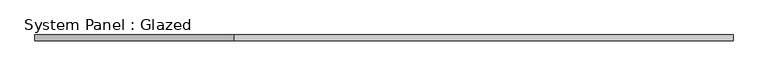
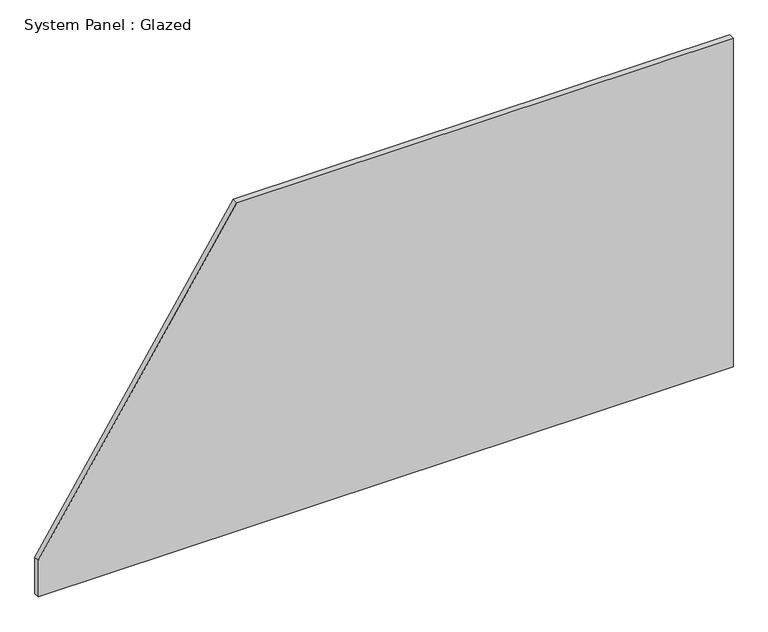
"""IFC4 building model written with IfcOpenShell, lengths in millimetres: plate geometry, System Panel : Glazed."""

from ifc_helpers import new_model, si_unit, frame, origin, place, context, project, spatial, polyline, outline, extrude, source, transform, mapped, element, save


def system_panel_glazed_b6f49b0a(model_context):
    return source(origin(), model_context, "Body", "SweptSolid", [
        extrude(outline(polyline([(0.0, -1500.0), (0.0, 1500.0), (1500.0, 1500.0), (1500.0, -642.8120991), (166.61217, -1500.0), (0.0, -1500.0)])), frame((0.0, 24.5, 0.0), z_axis=(0.0, 1.0, 0.0), x_axis=(0.0, 0.0, 1.0)), (0.0, 0.0, 1.0), 25.0),
    ])


if __name__ == "__main__":
    model = new_model("IFC4")
    model_context = context("Model", 3, world=origin())
    ifc_project = project(units=[si_unit("LENGTHUNIT", "METRE", prefix="MILLI")], contexts=[model_context])
    site = spatial("IfcSite", under=ifc_project)
    building = spatial("IfcBuilding", under=site)
    placement = place(None, origin())
    system_panel_glazed_shape = system_panel_glazed_b6f49b0a(model_context)
    element("IfcPlate", 1, ObjectType="System Panel : Glazed", at=placement, inside=building, context=model_context, shape_type="MappedRepresentation", body=[
        mapped(system_panel_glazed_shape, transform((0.0, 0.0, 0.0), x_axis=(1.0, 0.0, 0.0), y_axis=(0.0, 1.0, 0.0), z_axis=(0.0, 0.0, 1.0))),
    ])
    save(model, "model.ifc")

# Revit data of these elements
# Type "System Panel : Glazed"
#   Construction Type Id = "GSP4R"
#   Analytic Construction = "1/8 in Pilkington single glazing"
#   Visual Light Transmittance = 0.9
#   Solar Heat Gain Coefficient = 0.86
#   Heat Transfer Coefficient (U) = 6.7069 W/(m²·K)
#   Define Thermal Properties by = 1
# Element 1 (IfcPlate, "System Panel : Glazed")
#   Materials on its faces: "Glass"
# Materials
#   "Glass": class "Glass", colour RGB 0 128 192, transparency 0.9, Description = "Soda Lime Glass", Cost = 0
